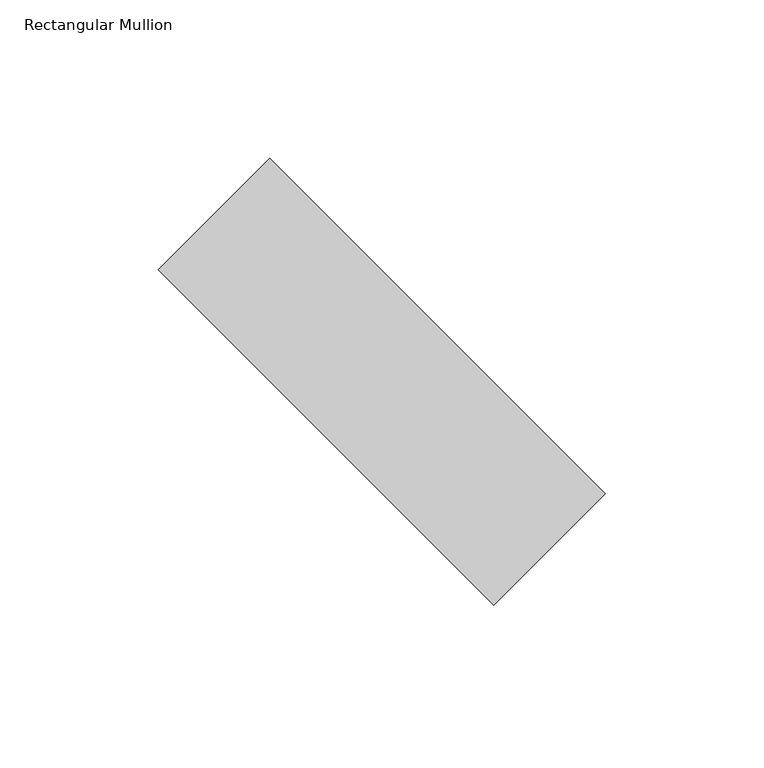
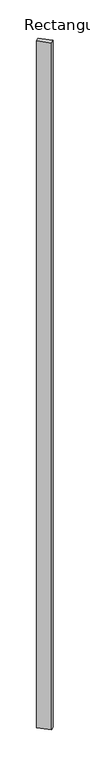
"""IFC4 building model written with IfcOpenShell, lengths in millimetres: member geometry, Rectangular Mullion : tilted mullions."""

import ifcopenshell
import ifcopenshell.guid

model = None  # the IFC model being written
_history = None  # IfcOwnerHistory: only IFC2X3 demands one
_inside = {}  # id of a spatial element -> (the spatial element, [elements in it])
_under = {}  # id of a project, library or spatial element -> (it, [spatial elements below it])
_declared = {}  # id of a project -> (the project, [libraries it declares])
_typed = {}  # id of a type object -> (the type object, [elements of that type])
_made_of = {}  # id of a material, layer set ... -> (it, [elements and type objects made of it])


def new_model(schema):
    """Start an empty IFC model of exactly this schema.

    Asked for "IFC4X3", IfcOpenShell would pick the latest addendum, in which some entities
    have other attributes; the version numbers below select the first issue.
    IFC2X3 requires an IfcOwnerHistory on every rooted entity: one is made here for all.
    """
    global model, _history
    if schema == "IFC4X3":
        model = ifcopenshell.file(schema_version=(4, 3, 0, 0))
    else:
        model = ifcopenshell.file(schema=schema)
    _inside.clear()
    _under.clear()
    _declared.clear()
    _typed.clear()
    _made_of.clear()
    _history = None
    if model.schema == "IFC2X3":
        org = make("IfcOrganization", Name="unknown")
        user = make(
            "IfcPersonAndOrganization",
            ThePerson=make("IfcPerson", FamilyName="unknown"),
            TheOrganization=org,
        )
        app = make(
            "IfcApplication",
            ApplicationDeveloper=org,
            Version="unknown",
            ApplicationFullName="unknown",
            ApplicationIdentifier="unknown",
        )
        _history = make(
            "IfcOwnerHistory",
            OwningUser=user,
            OwningApplication=app,
            ChangeAction="ADDED",
            CreationDate=0,
        )
    return model


def make(cls, **values):
    """One entity of the class cls with the attributes given. An attribute that is None is left unset."""
    return model.create_entity(
        cls, **{name: value for name, value in values.items() if value is not None}
    )


def rooted(cls, **values):
    """An entity with a GlobalId (a new one), such as an element, a storey or a relation."""
    return make(cls, GlobalId=ifcopenshell.guid.new(), OwnerHistory=_history, **values)


def si_unit(unit_type, name, prefix=None):
    """IfcSIUnit, for example si_unit("LENGTHUNIT", "METRE", prefix="MILLI")."""
    return make("IfcSIUnit", UnitType=unit_type, Prefix=prefix, Name=name)


def assignment(units):
    """IfcUnitAssignment: the units of a project."""
    return None if units is None else make("IfcUnitAssignment", Units=units)


def point(xyz):
    """IfcCartesianPoint."""
    return None if xyz is None else make("IfcCartesianPoint", Coordinates=xyz)


def direction(xyz):
    """IfcDirection."""
    return None if xyz is None else make("IfcDirection", DirectionRatios=xyz)


def frame(location, z_axis=None, x_axis=None):
    """IfcAxis2Placement3D, a coordinate frame: its origin and axes. An axis left out is left unset."""
    return make(
        "IfcAxis2Placement3D",
        Location=point(location),
        Axis=direction(z_axis),
        RefDirection=direction(x_axis),
    )


def origin():
    """The frame at (0, 0, 0) with its axes left unset."""
    return frame((0.0, 0.0, 0.0))


def place(relative_to, where):
    """IfcLocalPlacement: puts the frame where relative to a parent placement (None: the world)."""
    return make(
        "IfcLocalPlacement", PlacementRelTo=relative_to, RelativePlacement=where
    )


def context(
    kind, dimensions, precision=None, world=None, true_north=None, identifier=None
):
    """IfcGeometricRepresentationContext, for example the 3D "Model" context."""
    return make(
        "IfcGeometricRepresentationContext",
        ContextIdentifier=identifier,
        ContextType=kind,
        CoordinateSpaceDimension=dimensions,
        Precision=precision,
        WorldCoordinateSystem=world,
        TrueNorth=true_north,
    )


def project(units=None, contexts=None):
    """IfcProject with its units and contexts."""
    return rooted(
        "IfcProject",
        Name="project",
        RepresentationContexts=contexts,
        UnitsInContext=assignment(units),
    )


def spatial(cls, under=None, at=None, **own):
    """A site, building, storey or space (cls), placed at a placement, below another one or the project."""
    s = rooted(cls, ObjectPlacement=at, **own)
    if under is not None:
        _under.setdefault(under.id(), (under, []))[1].append(s)
    return s


def polyline(points):
    """IfcPolyline through the points."""
    return make("IfcPolyline", Points=[point(p) for p in points])


def outline(outer, holes=None, kind="AREA"):
    """IfcArbitraryClosedProfileDef: a profile drawn as a closed curve; with holes, ...WithVoids."""
    if holes is None:
        return make("IfcArbitraryClosedProfileDef", ProfileType=kind, OuterCurve=outer)
    return make(
        "IfcArbitraryProfileDefWithVoids",
        ProfileType=kind,
        OuterCurve=outer,
        InnerCurves=holes,
    )


def extrude(swept, where, along, depth):
    """IfcExtrudedAreaSolid: the profile swept, set in the frame where, extruded along a direction by depth."""
    return make(
        "IfcExtrudedAreaSolid",
        SweptArea=swept,
        Position=where,
        ExtrudedDirection=direction(along),
        Depth=depth,
    )


def shape(context_of_items, identifier, shape_type, items):
    """IfcShapeRepresentation: the items that make up one representation, for example the "Body"."""
    return make(
        "IfcShapeRepresentation",
        ContextOfItems=context_of_items,
        RepresentationIdentifier=identifier,
        RepresentationType=shape_type,
        Items=items,
    )


def source(mapping_origin, context_of_items, identifier, shape_type, items):
    """IfcRepresentationMap: a shape defined once, which mapped items show again and again."""
    return make(
        "IfcRepresentationMap",
        MappingOrigin=mapping_origin,
        MappedRepresentation=shape(context_of_items, identifier, shape_type, items),
    )


def transform(
    local_origin,
    x_axis=None,
    y_axis=None,
    z_axis=None,
    scale=None,
    scale2=None,
    scale3=None,
    uniform=True,
):
    """IfcCartesianTransformationOperator3D, or its non-uniform kind. x_axis, y_axis, z_axis: its Axis1, 2, 3."""
    if uniform:
        return make(
            "IfcCartesianTransformationOperator3D",
            Axis1=direction(x_axis),
            Axis2=direction(y_axis),
            LocalOrigin=point(local_origin),
            Scale=scale,
            Axis3=direction(z_axis),
        )
    return make(
        "IfcCartesianTransformationOperator3DnonUniform",
        Axis1=direction(x_axis),
        Axis2=direction(y_axis),
        LocalOrigin=point(local_origin),
        Scale=scale,
        Axis3=direction(z_axis),
        Scale2=scale2,
        Scale3=scale3,
    )


def mapped(mapping_source, mapping_target):
    """IfcMappedItem: shows the shape of a source again, moved by a transform."""
    return make(
        "IfcMappedItem", MappingSource=mapping_source, MappingTarget=mapping_target
    )


def made_of(thing, what):
    """Note that an element or type object is made of a material, layer set ...; save() writes the relation."""
    if what is not None:
        _made_of.setdefault(what.id(), (what, []))[1].append(thing)
    return thing


def element(
    cls,
    number,
    at=None,
    inside=None,
    cuts=None,
    type_object=None,
    material=None,
    context=None,
    identifier="Body",
    shape_type=None,
    held_by="IfcProductDefinitionShape",
    body=None,
    shapes=None,
    **own,
):
    """One element of the class cls, such as IfcWall. Its Tag is "e" and its number.

    at: its placement. inside: the storey or other place that contains it. cuts: it is an
    opening in that element (IfcRelVoidsElement). A single representation is given by context,
    identifier, shape_type and body (its items); several are given by shapes. held_by: the class
    of the entity that holds the representations. save() writes the other relations.
    """
    e = rooted(cls, Tag="e%d" % number, ObjectPlacement=at, **own)
    if body is not None:
        shapes = [shape(context, identifier, shape_type, body)]
    if shapes is not None:
        e.Representation = make(held_by, Representations=shapes)
    if inside is not None:
        _inside.setdefault(inside.id(), (inside, []))[1].append(e)
    if cuts is not None:
        rooted(
            "IfcRelVoidsElement", RelatingBuildingElement=cuts, RelatedOpeningElement=e
        )
    if type_object is not None:
        _typed.setdefault(type_object.id(), (type_object, []))[1].append(e)
    return made_of(e, material)


def aggregate(whole, parts):
    """IfcRelAggregates: a whole, such as a stair, and the parts it consists of."""
    return rooted("IfcRelAggregates", RelatingObject=whole, RelatedObjects=parts)


def save(model, path):
    """Write the relations noted so far, then the file.

    IfcRelAggregates (storeys below a building ...), IfcRelContainedInSpatialStructure (elements
    in a storey), IfcRelDefinesByType, IfcRelAssociatesMaterial and IfcRelDeclares: one each for
    every whole, place, type object, material and project.
    """
    for whole, parts in _under.values():
        aggregate(whole, parts)
    for where, things in _inside.values():
        rooted(
            "IfcRelContainedInSpatialStructure",
            RelatedElements=things,
            RelatingStructure=where,
        )
    for kind, things in _typed.values():
        rooted("IfcRelDefinesByType", RelatedObjects=things, RelatingType=kind)
    for what, things in _made_of.values():
        rooted("IfcRelAssociatesMaterial", RelatedObjects=things, RelatingMaterial=what)
    for by, libraries in _declared.values():
        rooted("IfcRelDeclares", RelatingContext=by, RelatedDefinitions=libraries)
    model.write(path)


def rectangular_mullion_0e496170(model_context):
    return source(origin(), model_context, "Body", "SweptSolid", [
        extrude(outline(polyline([(-35.3553391, 70.7106781), (70.7106781, -35.3553391), (35.3553391, -70.7106781), (-70.7106781, 35.3553391), (-35.3553391, 70.7106781)])), frame((0.0, 0.0, -8000.0002611), z_axis=(0.0, 0.0, 1.0), x_axis=(1.0, 0.0, 0.0)), (0.0, 0.0, 1.0), 8000.0002611),
    ])


if __name__ == "__main__":
    model = new_model("IFC4")
    model_context = context("Model", 3, world=origin())
    ifc_project = project(units=[si_unit("LENGTHUNIT", "METRE", prefix="MILLI")], contexts=[model_context])
    site = spatial("IfcSite", under=ifc_project)
    building = spatial("IfcBuilding", under=site)
    placement = place(None, origin())
    rectangular_mullion_shape = rectangular_mullion_0e496170(model_context)
    element("IfcMember", 1, ObjectType="Rectangular Mullion : tilted mullions", at=placement, inside=building, context=model_context, shape_type="MappedRepresentation", body=[
        mapped(rectangular_mullion_shape, transform((0.0, 0.0, 0.0), x_axis=(1.0, 0.0, 0.0), y_axis=(0.0, 1.0, 0.0), z_axis=(0.0, 0.0, 1.0))),
    ])
    save(model, "model.ifc")

# Revit data of these elements
# Project information
#   Project Issue Date = "Issue Date"
#   Project Status = "Project  Status"
#   Client Name = "Owner"
#   Project Address = "## Street\nCity, State  Zip"
#   Project Name = "Project Name"
#   Project Number = "Project  Number"
# Type "Rectangular Mullion : tilted mullions"
#   built-in parameter 1007304 = 0.492126 (stored number, unit not read)
#   built-in parameter 1007301 = 0.082021 (stored number, unit not read)
#   built-in parameter 1007300 = 0.082021 (stored number, unit not read)
# Element 1 (IfcMember, "Rectangular Mullion : tilted mullions")
#   Materials on its faces: "Aluminum"
# Materials
#   "Aluminum": class "Metal", colour RGB 244 244 244, transparency 0, Description = "Aluminum 6061", Cost = 0
